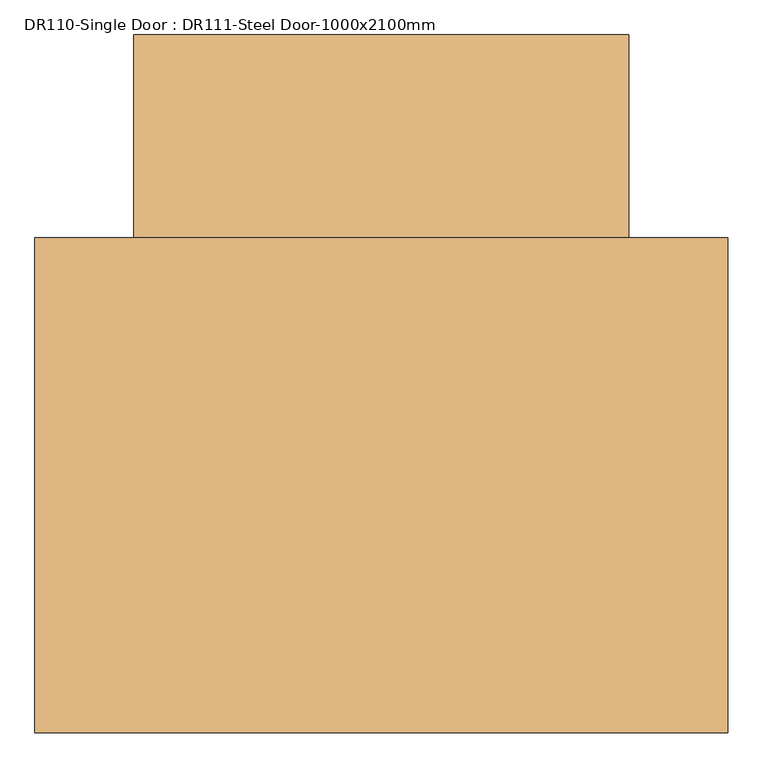
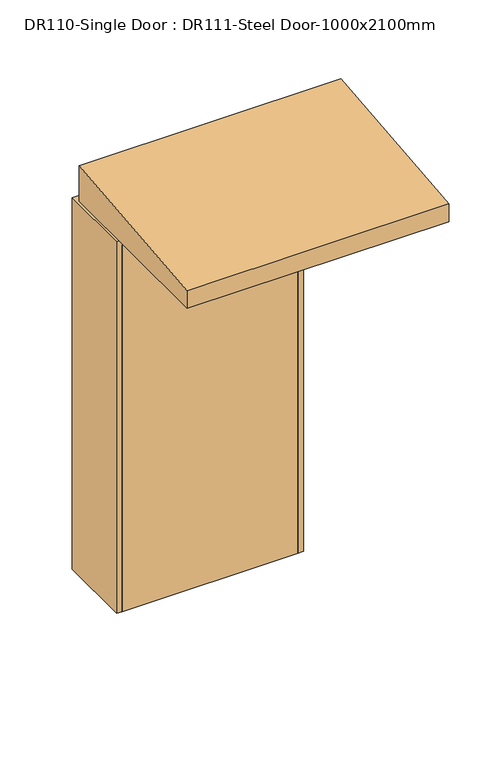
"""IFC4 building model written with IfcOpenShell, lengths in millimetres: door geometry, DR110-Single Door : DR111-Steel Door-1000x2100mm."""

import ifcopenshell
import ifcopenshell.guid

model = None  # the IFC model being written
_history = None  # IfcOwnerHistory: only IFC2X3 demands one
_inside = {}  # id of a spatial element -> (the spatial element, [elements in it])
_under = {}  # id of a project, library or spatial element -> (it, [spatial elements below it])
_declared = {}  # id of a project -> (the project, [libraries it declares])
_typed = {}  # id of a type object -> (the type object, [elements of that type])
_made_of = {}  # id of a material, layer set ... -> (it, [elements and type objects made of it])


def new_model(schema):
    """Start an empty IFC model of exactly this schema.

    Asked for "IFC4X3", IfcOpenShell would pick the latest addendum, in which some entities
    have other attributes; the version numbers below select the first issue.
    IFC2X3 requires an IfcOwnerHistory on every rooted entity: one is made here for all.
    """
    global model, _history
    if schema == "IFC4X3":
        model = ifcopenshell.file(schema_version=(4, 3, 0, 0))
    else:
        model = ifcopenshell.file(schema=schema)
    _inside.clear()
    _under.clear()
    _declared.clear()
    _typed.clear()
    _made_of.clear()
    _history = None
    if model.schema == "IFC2X3":
        org = make("IfcOrganization", Name="unknown")
        user = make(
            "IfcPersonAndOrganization",
            ThePerson=make("IfcPerson", FamilyName="unknown"),
            TheOrganization=org,
        )
        app = make(
            "IfcApplication",
            ApplicationDeveloper=org,
            Version="unknown",
            ApplicationFullName="unknown",
            ApplicationIdentifier="unknown",
        )
        _history = make(
            "IfcOwnerHistory",
            OwningUser=user,
            OwningApplication=app,
            ChangeAction="ADDED",
            CreationDate=0,
        )
    return model


def make(cls, **values):
    """One entity of the class cls with the attributes given. An attribute that is None is left unset."""
    return model.create_entity(
        cls, **{name: value for name, value in values.items() if value is not None}
    )


def rooted(cls, **values):
    """An entity with a GlobalId (a new one), such as an element, a storey or a relation."""
    return make(cls, GlobalId=ifcopenshell.guid.new(), OwnerHistory=_history, **values)


def si_unit(unit_type, name, prefix=None):
    """IfcSIUnit, for example si_unit("LENGTHUNIT", "METRE", prefix="MILLI")."""
    return make("IfcSIUnit", UnitType=unit_type, Prefix=prefix, Name=name)


def assignment(units):
    """IfcUnitAssignment: the units of a project."""
    return None if units is None else make("IfcUnitAssignment", Units=units)


def point(xyz):
    """IfcCartesianPoint."""
    return None if xyz is None else make("IfcCartesianPoint", Coordinates=xyz)


def direction(xyz):
    """IfcDirection."""
    return None if xyz is None else make("IfcDirection", DirectionRatios=xyz)


def frame(location, z_axis=None, x_axis=None):
    """IfcAxis2Placement3D, a coordinate frame: its origin and axes. An axis left out is left unset."""
    return make(
        "IfcAxis2Placement3D",
        Location=point(location),
        Axis=direction(z_axis),
        RefDirection=direction(x_axis),
    )


def origin():
    """The frame at (0, 0, 0) with its axes left unset."""
    return frame((0.0, 0.0, 0.0))


def origin_with_axes():
    """The frame at (0, 0, 0) with the z axis (0, 0, 1) and the x axis (1, 0, 0) written out."""
    return frame((0.0, 0.0, 0.0), z_axis=(0.0, 0.0, 1.0), x_axis=(1.0, 0.0, 0.0))


def place(relative_to, where):
    """IfcLocalPlacement: puts the frame where relative to a parent placement (None: the world)."""
    return make(
        "IfcLocalPlacement", PlacementRelTo=relative_to, RelativePlacement=where
    )


def context(
    kind, dimensions, precision=None, world=None, true_north=None, identifier=None
):
    """IfcGeometricRepresentationContext, for example the 3D "Model" context."""
    return make(
        "IfcGeometricRepresentationContext",
        ContextIdentifier=identifier,
        ContextType=kind,
        CoordinateSpaceDimension=dimensions,
        Precision=precision,
        WorldCoordinateSystem=world,
        TrueNorth=true_north,
    )


def project(units=None, contexts=None):
    """IfcProject with its units and contexts."""
    return rooted(
        "IfcProject",
        Name="project",
        RepresentationContexts=contexts,
        UnitsInContext=assignment(units),
    )


def spatial(cls, under=None, at=None, **own):
    """A site, building, storey or space (cls), placed at a placement, below another one or the project."""
    s = rooted(cls, ObjectPlacement=at, **own)
    if under is not None:
        _under.setdefault(under.id(), (under, []))[1].append(s)
    return s


def polyline(points):
    """IfcPolyline through the points."""
    return make("IfcPolyline", Points=[point(p) for p in points])


def outline(outer, holes=None, kind="AREA"):
    """IfcArbitraryClosedProfileDef: a profile drawn as a closed curve; with holes, ...WithVoids."""
    if holes is None:
        return make("IfcArbitraryClosedProfileDef", ProfileType=kind, OuterCurve=outer)
    return make(
        "IfcArbitraryProfileDefWithVoids",
        ProfileType=kind,
        OuterCurve=outer,
        InnerCurves=holes,
    )


def extrude(swept, where, along, depth):
    """IfcExtrudedAreaSolid: the profile swept, set in the frame where, extruded along a direction by depth."""
    return make(
        "IfcExtrudedAreaSolid",
        SweptArea=swept,
        Position=where,
        ExtrudedDirection=direction(along),
        Depth=depth,
    )


def faces_of(points, faces, orient=None, outer=None):
    """IfcFace entities. A face is a list of loops; a loop is a list of indices into points, from 0.

    orient and outer hold one flag for each loop. By default every Orientation is true, the
    first loop of a face is its IfcFaceOuterBound and the others are IfcFaceBound.
    """
    made = []
    for i, loops in enumerate(faces):
        bounds = []
        for j, loop in enumerate(loops):
            is_outer = j == 0 if outer is None else outer[i][j]
            bounds.append(
                make(
                    "IfcFaceOuterBound" if is_outer else "IfcFaceBound",
                    Bound=make("IfcPolyLoop", Polygon=[points[k] for k in loop]),
                    Orientation=True if orient is None else orient[i][j],
                )
            )
        made.append(make("IfcFace", Bounds=bounds))
    return made


def faceted_brep(points, faces, orient=None, outer=None, voids=None):
    """IfcFacetedBrep: a solid bounded by flat faces; with voids (closed shells), ...WithVoids."""
    shared = [point(p) for p in points]
    hull = make("IfcClosedShell", CfsFaces=faces_of(shared, faces, orient, outer))
    if voids is None:
        return make("IfcFacetedBrep", Outer=hull)
    return make(
        "IfcFacetedBrepWithVoids",
        Outer=hull,
        Voids=[
            make(cls, CfsFaces=faces_of(shared, fs, o, b)) for cls, fs, o, b in voids
        ],
    )


def shape(context_of_items, identifier, shape_type, items):
    """IfcShapeRepresentation: the items that make up one representation, for example the "Body"."""
    return make(
        "IfcShapeRepresentation",
        ContextOfItems=context_of_items,
        RepresentationIdentifier=identifier,
        RepresentationType=shape_type,
        Items=items,
    )


def source(mapping_origin, context_of_items, identifier, shape_type, items):
    """IfcRepresentationMap: a shape defined once, which mapped items show again and again."""
    return make(
        "IfcRepresentationMap",
        MappingOrigin=mapping_origin,
        MappedRepresentation=shape(context_of_items, identifier, shape_type, items),
    )


def transform(
    local_origin,
    x_axis=None,
    y_axis=None,
    z_axis=None,
    scale=None,
    scale2=None,
    scale3=None,
    uniform=True,
):
    """IfcCartesianTransformationOperator3D, or its non-uniform kind. x_axis, y_axis, z_axis: its Axis1, 2, 3."""
    if uniform:
        return make(
            "IfcCartesianTransformationOperator3D",
            Axis1=direction(x_axis),
            Axis2=direction(y_axis),
            LocalOrigin=point(local_origin),
            Scale=scale,
            Axis3=direction(z_axis),
        )
    return make(
        "IfcCartesianTransformationOperator3DnonUniform",
        Axis1=direction(x_axis),
        Axis2=direction(y_axis),
        LocalOrigin=point(local_origin),
        Scale=scale,
        Axis3=direction(z_axis),
        Scale2=scale2,
        Scale3=scale3,
    )


def mapped(mapping_source, mapping_target):
    """IfcMappedItem: shows the shape of a source again, moved by a transform."""
    return make(
        "IfcMappedItem", MappingSource=mapping_source, MappingTarget=mapping_target
    )


def made_of(thing, what):
    """Note that an element or type object is made of a material, layer set ...; save() writes the relation."""
    if what is not None:
        _made_of.setdefault(what.id(), (what, []))[1].append(thing)
    return thing


def element(
    cls,
    number,
    at=None,
    inside=None,
    cuts=None,
    type_object=None,
    material=None,
    context=None,
    identifier="Body",
    shape_type=None,
    held_by="IfcProductDefinitionShape",
    body=None,
    shapes=None,
    **own,
):
    """One element of the class cls, such as IfcWall. Its Tag is "e" and its number.

    at: its placement. inside: the storey or other place that contains it. cuts: it is an
    opening in that element (IfcRelVoidsElement). A single representation is given by context,
    identifier, shape_type and body (its items); several are given by shapes. held_by: the class
    of the entity that holds the representations. save() writes the other relations.
    """
    e = rooted(cls, Tag="e%d" % number, ObjectPlacement=at, **own)
    if body is not None:
        shapes = [shape(context, identifier, shape_type, body)]
    if shapes is not None:
        e.Representation = make(held_by, Representations=shapes)
    if inside is not None:
        _inside.setdefault(inside.id(), (inside, []))[1].append(e)
    if cuts is not None:
        rooted(
            "IfcRelVoidsElement", RelatingBuildingElement=cuts, RelatedOpeningElement=e
        )
    if type_object is not None:
        _typed.setdefault(type_object.id(), (type_object, []))[1].append(e)
    return made_of(e, material)


def aggregate(whole, parts):
    """IfcRelAggregates: a whole, such as a stair, and the parts it consists of."""
    return rooted("IfcRelAggregates", RelatingObject=whole, RelatedObjects=parts)


def save(model, path):
    """Write the relations noted so far, then the file.

    IfcRelAggregates (storeys below a building ...), IfcRelContainedInSpatialStructure (elements
    in a storey), IfcRelDefinesByType, IfcRelAssociatesMaterial and IfcRelDeclares: one each for
    every whole, place, type object, material and project.
    """
    for whole, parts in _under.values():
        aggregate(whole, parts)
    for where, things in _inside.values():
        rooted(
            "IfcRelContainedInSpatialStructure",
            RelatedElements=things,
            RelatingStructure=where,
        )
    for kind, things in _typed.values():
        rooted("IfcRelDefinesByType", RelatedObjects=things, RelatingType=kind)
    for what, things in _made_of.values():
        rooted("IfcRelAssociatesMaterial", RelatedObjects=things, RelatingMaterial=what)
    for by, libraries in _declared.values():
        rooted("IfcRelDeclares", RelatingContext=by, RelatedDefinitions=libraries)
    model.write(path)


def dr110_single_door_dr111_steel_door_1000x2100mm_4484fb18(model_context):
    return source(origin(), model_context, "Body", "SolidModel", [
        extrude(outline(polyline([(470.0, -205.0), (-470.0, -205.0), (-470.0, -170.0), (470.0, -170.0), (470.0, -205.0)])), origin_with_axes(), (0.0, 0.0, 1.0), 2070.0),
        faceted_brep([(470.0, -205.0, 0.0), (470.0, -170.0, 0.0), (450.0, -170.0, 0.0), (450.0, 170.0, 0.0), (470.0, 170.0, 0.0), (470.0, 205.0, 0.0), (500.0, 205.0, 0.0), (500.0, -205.0, 0.0), (500.0, -205.0, 2100.0), (-500.0, -205.0, 2100.0), (-500.0, -205.0, 0.0), (-470.0, -205.0, 0.0), (-470.0, -205.0, 2070.0), (470.0, -205.0, 2070.0), (500.0, 205.0, 2100.0), (470.0, 205.0, 2070.0), (-470.0, 205.0, 2070.0), (-470.0, 205.0, 0.0), (-500.0, 205.0, 0.0), (-500.0, 205.0, 2100.0), (470.0, 170.0, 2070.0), (450.0, 170.0, 2050.0), (-450.0, 170.0, 2050.0), (-450.0, 170.0, 0.0), (-470.0, 170.0, 0.0), (-470.0, 170.0, 2070.0), (450.0, -170.0, 2050.0), (470.0, -170.0, 2070.0), (-470.0, -170.0, 2070.0), (-470.0, -170.0, 0.0), (-450.0, -170.0, 0.0), (-450.0, -170.0, 2050.0)], [[[0, 1, 2, 3, 4, 5, 6, 7]], [[7, 8, 9, 10, 11, 12, 13, 0]], [[6, 14, 8, 7]], [[5, 15, 16, 17, 18, 19, 14, 6]], [[4, 20, 15, 5]], [[3, 21, 22, 23, 24, 25, 20, 4]], [[2, 26, 21, 3]], [[1, 27, 28, 29, 30, 31, 26, 2]], [[0, 13, 27, 1]], [[12, 11, 29, 28]], [[11, 10, 18, 17, 24, 23, 30, 29]], [[19, 18, 10, 9]], [[25, 24, 17, 16]], [[31, 30, 23, 22]], [[14, 19, 9, 8]], [[20, 25, 16, 15]], [[26, 31, 22, 21]], [[13, 12, 28, 27]]]),
        extrude(outline(polyline([(-1205.0, 2400.0), (-1205.0, 2500.0), (-205.0, 2600.0), (-205.0, 2400.0), (-1205.0, 2400.0)])), frame((-700.0, 0.0, 0.0), z_axis=(1.0, 0.0, 0.0), x_axis=(0.0, 1.0, 0.0)), (0.0, 0.0, 1.0), 1400.0),
    ])


if __name__ == "__main__":
    model = new_model("IFC4")
    model_context = context("Model", 3, world=origin())
    ifc_project = project(units=[si_unit("LENGTHUNIT", "METRE", prefix="MILLI")], contexts=[model_context])
    site = spatial("IfcSite", under=ifc_project)
    building = spatial("IfcBuilding", under=site)
    placement = place(None, origin())
    dr110_single_door_dr111_steel_door_1000x2100mm_shape = dr110_single_door_dr111_steel_door_1000x2100mm_4484fb18(model_context)
    element("IfcDoor", 1, ObjectType="DR110-Single Door : DR111-Steel Door-1000x2100mm", at=placement, inside=building, context=model_context, shape_type="MappedRepresentation", body=[
        mapped(dr110_single_door_dr111_steel_door_1000x2100mm_shape, transform((0.0, 0.0, 0.0), x_axis=(1.0, 0.0, 0.0), y_axis=(0.0, 1.0, 0.0), z_axis=(0.0, 0.0, 1.0))),
    ])
    save(model, "model.ifc")

# Revit data of these elements
# Type "DR110-Single Door : DR111-Steel Door-1000x2100mm"
#   Type Mark = "SD"
#   Analytic Construction = "<None>"
#   프레임 투영 외부. = 25 mm
#   프레임 투영 내부. = 25 mm
#   프레임 폭 = 75 mm
#   Height = 2100 mm
#   Width = 1000 mm
#   Define Thermal Properties by = 1
#   Canopy [instance default] = yes
#   문 패널 = SD1 문 패널
#   문 프레임 = A04AQ098-00002_Steel Door_non FP_single
#   Function = (empty or 0)
#   Wall Closure = (empty or 0)
# Element 1 (IfcDoor, "DR110-Single Door : DR111-Steel Door-1000x2100mm")
#   Materials on its faces: "A04AQ098-00002_Steel Door_non FP_single", "SD1 문 패널"
# Materials
#   "SD1 문 패널": class "금속", colour RGB 247 247 247, transparency 0
#   "A04AQ098-00002_Steel Door_non FP_single": class "금속", colour RGB 247 247 247, transparency 0, Description = "Steel Door", W00) Work Master Code = "A04AQ098-00002", W01) Work Master_Lv1 = "Finishing Work", W02) Work Master_Lv2 = "Door & Window Work", W03) Work Master_Spec.1 = "Steel Door w/ Steel Frame", W04) Work Master_Spec.2 = "Fire Protective Rating: N/A, Single Door", W05) Work Master_Spec.3 = "w/ Hardware & Accessories", Cost = 0
